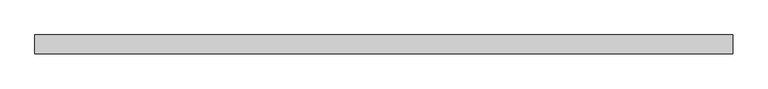
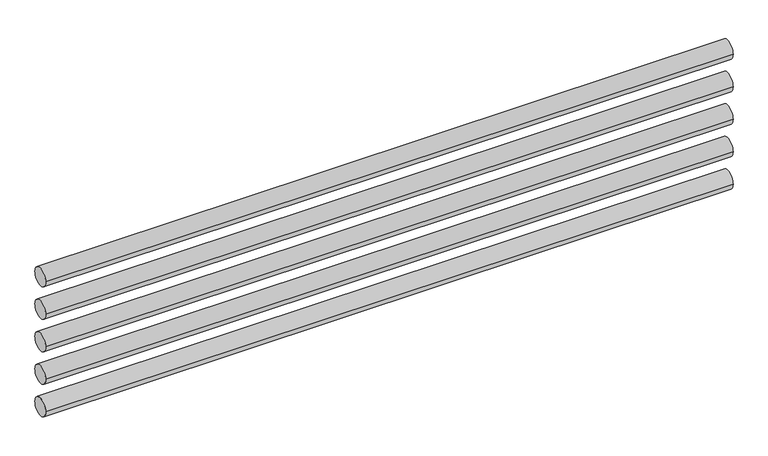
"""IFC4 building model written with IfcOpenShell, lengths in millimetres: proxy geometry, Газпремиум_Регистр : РГТ-1-108х3-4м-5."""

from ifc_helpers import new_model, si_unit, point, frame, frame_2d, origin, place, context, project, spatial, circle_curve, trimmed, segment, composite_curve, outline, extrude, source, transform, mapped, element, save


def mechanical_equipment_0d4bc756(model_context):
    return source(origin(), model_context, "Body", "SweptSolid", [
        extrude(outline(composite_curve([segment(trimmed(circle_curve(frame_2d((0.0, 854.0)), 54.0), [point((-54.0, 854.0))], [point((54.0, 854.0))], False, "CARTESIAN"), True, "CONTINUOUS"), segment(trimmed(circle_curve(frame_2d((0.0, 854.0)), 54.0), [point((54.0, 854.0))], [point((-54.0, 854.0))], False, "CARTESIAN"), True, "CONTINUOUS")], self_intersect=False)), frame((-1184.1719207, 0.0, 0.0), z_axis=(1.0, 0.0, 0.0), x_axis=(0.0, 1.0, 0.0)), (0.0, 0.0, 1.0), 4000.0),
        extrude(outline(composite_curve([segment(trimmed(circle_curve(frame_2d((0.0, 654.0)), 54.0), [point((-54.0, 654.0))], [point((54.0, 654.0))], False, "CARTESIAN"), True, "CONTINUOUS"), segment(trimmed(circle_curve(frame_2d((0.0, 654.0)), 54.0), [point((54.0, 654.0))], [point((-54.0, 654.0))], False, "CARTESIAN"), True, "CONTINUOUS")], self_intersect=False)), frame((-1184.1719207, 0.0, 0.0), z_axis=(1.0, 0.0, 0.0), x_axis=(0.0, 1.0, 0.0)), (0.0, 0.0, 1.0), 4000.0),
        extrude(outline(composite_curve([segment(trimmed(circle_curve(frame_2d((0.0, 454.0)), 54.0), [point((-54.0, 454.0))], [point((54.0, 454.0))], False, "CARTESIAN"), True, "CONTINUOUS"), segment(trimmed(circle_curve(frame_2d((0.0, 454.0)), 54.0), [point((54.0, 454.0))], [point((-54.0, 454.0))], False, "CARTESIAN"), True, "CONTINUOUS")], self_intersect=False)), frame((-1184.1719207, 0.0, 0.0), z_axis=(1.0, 0.0, 0.0), x_axis=(0.0, 1.0, 0.0)), (0.0, 0.0, 1.0), 4000.0),
        extrude(outline(composite_curve([segment(trimmed(circle_curve(frame_2d((0.0, 254.0)), 54.0), [point((-54.0, 254.0))], [point((54.0, 254.0))], False, "CARTESIAN"), True, "CONTINUOUS"), segment(trimmed(circle_curve(frame_2d((0.0, 254.0)), 54.0), [point((54.0, 254.0))], [point((-54.0, 254.0))], False, "CARTESIAN"), True, "CONTINUOUS")], self_intersect=False)), frame((-1184.1719207, 0.0, 0.0), z_axis=(1.0, 0.0, 0.0), x_axis=(0.0, 1.0, 0.0)), (0.0, 0.0, 1.0), 4000.0),
        extrude(outline(composite_curve([segment(trimmed(circle_curve(frame_2d((0.0, 54.0)), 54.0), [point((-54.0, 54.0))], [point((54.0, 54.0))], False, "CARTESIAN"), True, "CONTINUOUS"), segment(trimmed(circle_curve(frame_2d((0.0, 54.0)), 54.0), [point((54.0, 54.0))], [point((-54.0, 54.0))], False, "CARTESIAN"), True, "CONTINUOUS")], self_intersect=False)), frame((-1184.1719207, 0.0, 0.0), z_axis=(1.0, 0.0, 0.0), x_axis=(0.0, 1.0, 0.0)), (0.0, 0.0, 1.0), 4000.0),
    ])


if __name__ == "__main__":
    model = new_model("IFC4")
    model_context = context("Model", 3, world=origin())
    ifc_project = project(units=[si_unit("LENGTHUNIT", "METRE", prefix="MILLI")], contexts=[model_context])
    site = spatial("IfcSite", under=ifc_project)
    building = spatial("IfcBuilding", under=site)
    placement = place(None, origin())
    mechanical_equipment_shape = mechanical_equipment_0d4bc756(model_context)
    element("IfcBuildingElementProxy", 1, Name="Газпремиум_Регистр : РГТ-1-108х3-4м-5", ObjectType="Газпремиум_Регистр : РГТ-1-108х3-4м-5", at=placement, inside=building, context=model_context, shape_type="MappedRepresentation", body=[
        mapped(mechanical_equipment_shape, transform((0.0, 0.0, 0.0), x_axis=(1.0, 0.0, 0.0), y_axis=(0.0, 1.0, 0.0), z_axis=(0.0, 0.0, 1.0))),
    ])
    save(model, "model.ifc")

# Revit data of these elements
# Type "Газпремиум_Регистр : РГТ-1-108х3-4м-5"
#   ADSK_Позиция = "386"
#   ADSK_Наименование = "Регистр однорядный из пяти гладких труб 108х3 длиной 4 м, в комплекте с опорами"
#   ADSK_Марка = "РГТ-1-108х3-4м-5-ОП-О ТУ 4936-001-69441315-11"
#   ADSK_Код изделия = "2050906"
#   ADSK_Завод-изготовитель = "ООО ПКП \"ГазПремиум\", Россия, г.Саратов, ИНН 6452951387, кпп 645201001, gaz-premium@mail.ru"
#   ADSK_Единица измерения = "шт."
#   Расстояние между рядами = 200 mm
#   Радиус.регистра = 54 mm
#   Отступ.труб.подкл.от.осевой = 32.719 mm
#   Длина регистра = 4000 mm
#   Диаметр.труб.подкл. = 32 mm
#   Диаметр регистра = 108 mm
#   Высота = 800 mm
#   ADSK_Масса = 214.9
#   ADSK_Количество = 1
#   Число рядов = 5
#   Соед.трубы = Грунтовка.красная
#   Регистр = Грунтовка.красная
#   Поддерж.арматура = Грунтовка.серая
#   Default Elevation = 0
# Element 1 (IfcBuildingElementProxy, "Газпремиум_Регистр : РГТ-1-108х3-4м-5")
#   Materials on its faces: "Грунтовка.красная"
# Materials
#   "Грунтовка.красная": class "Разное", colour RGB 255 0 0, transparency 0
#   "Грунтовка.серая": class "Разное", colour RGB 187 181 179, transparency 0
